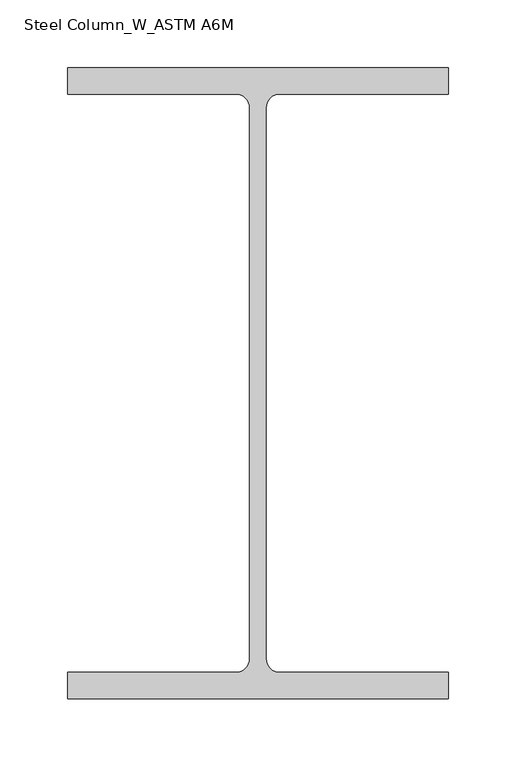
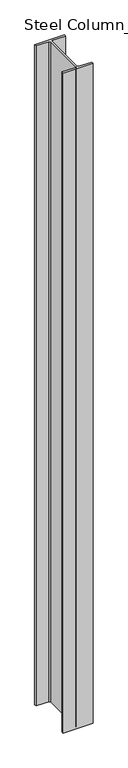
"""IFC4 building model written with IfcOpenShell, lengths in millimetres: column geometry, Steel Column_W_ASTM A6M : H_SC_AR_S01_W460x128_C1."""

from ifc_helpers import new_model, si_unit, point, frame, frame_2d, origin, place, context, project, spatial, polyline, circle_curve, trimmed, segment, composite_curve, outline, extrude, source, transform, mapped, element, save


def steel_column_w_astm_a6m_377c25c9(model_context):
    return source(origin(), model_context, "Body", "SweptSolid", [
        extrude(outline(composite_curve([segment(polyline([(141.0, 233.5), (141.0, 213.9), (16.2, 213.9)]), True, "CONTINUOUS"), segment(trimmed(circle_curve(frame_2d((16.2, 203.8)), 10.1), [point((16.2, 213.9))], [point((6.1, 203.8))], True, "CARTESIAN"), True, "CONTINUOUS"), segment(polyline([(6.1, 203.8), (6.1, -203.8)]), True, "CONTINUOUS"), segment(trimmed(circle_curve(frame_2d((16.2, -203.8)), 10.1), [point((6.1, -203.8))], [point((16.2, -213.9))], True, "CARTESIAN"), True, "CONTINUOUS"), segment(polyline([(16.2, -213.9), (141.0, -213.9), (141.0, -233.5), (-141.0, -233.5), (-141.0, -213.9), (-16.2, -213.9)]), True, "CONTINUOUS"), segment(trimmed(circle_curve(frame_2d((-16.2, -203.8)), 10.1), [point((-16.2, -213.9))], [point((-6.1, -203.8))], True, "CARTESIAN"), True, "CONTINUOUS"), segment(polyline([(-6.1, -203.8), (-6.1, 203.8)]), True, "CONTINUOUS"), segment(trimmed(circle_curve(frame_2d((-16.2, 203.8)), 10.1), [point((-6.1, 203.8))], [point((-16.2, 213.9))], True, "CARTESIAN"), True, "CONTINUOUS"), segment(polyline([(-16.2, 213.9), (-141.0, 213.9), (-141.0, 233.5), (141.0, 233.5)]), True, "CONTINUOUS")], self_intersect=False)), frame((0.0, 0.0, 3519.8243501), z_axis=(0.0, 0.0, 1.0), x_axis=(1.0, 0.0, 0.0)), (0.0, 0.0, 1.0), 6600.0),
    ])


if __name__ == "__main__":
    model = new_model("IFC4")
    model_context = context("Model", 3, world=origin())
    ifc_project = project(units=[si_unit("LENGTHUNIT", "METRE", prefix="MILLI")], contexts=[model_context])
    site = spatial("IfcSite", under=ifc_project)
    building = spatial("IfcBuilding", under=site)
    placement = place(None, origin())
    steel_column_w_astm_a6m_shape = steel_column_w_astm_a6m_377c25c9(model_context)
    element("IfcColumn", 1, ObjectType="Steel Column_W_ASTM A6M : H_SC_AR_S01_W460x128_C1", at=placement, inside=building, context=model_context, shape_type="MappedRepresentation", body=[
        mapped(steel_column_w_astm_a6m_shape, transform((0.0, 0.0, 0.0), x_axis=(1.0, 0.0, 0.0), y_axis=(0.0, 1.0, 0.0), z_axis=(0.0, 0.0, 1.0))),
    ])
    save(model, "model.ifc")

# Revit data of these elements
# Type "Steel Column_W_ASTM A6M : H_SC_AR_S01_W460x128_C1"
#   Section Name Key = "W18x86"
#   Width = 28.2 cm
#   Web Thickness = 1.22 cm
#   Web Fillet = 1.01 cm
#   Warping Constant = 3650000.0 cm⁶
#   Torsional Moment of Inertia = 171.00 cm⁴
#   Section Area = 163.0 cm²
#   Plastic Modulus weak axis = 793.0 cm³
#   Plastic Modulus strong axis = 3050.0 cm³
#   Perimeter = 2.02 m²/m
#   Nominal Weight = 128.00 kgf/m
#   Moment of Inertia weak axis = 7280.00 cm⁴
#   Moment of Inertia strong axis = 63700.00 cm⁴
#   Height = 46.7 cm
#   Flange Thickness = 1.96 cm
#   Elastic Modulus weak axis = 518.0 cm³
#   Elastic Modulus strong axis = 2720.0 cm³
#   Centroid Vertical = 23.35 cm
#   Centroid Horizontal = 14.1 cm
#   Structural Material [instance default] = Steel, 45-345
#   Bolt Spacing = 0
#   Assembly Code = ""
# Element 1 (IfcColumn, "Steel Column_W_ASTM A6M : H_SC_AR_S01_W460x128_C1")
#   Structural Material = Steel ASTM A992 GRADE 50
#   Materials on its faces: "Steel ASTM A992 GRADE 50"
# Materials
#   "Steel, 45-345": class "Metal", colour RGB 189 187 185, transparency 0, Description = "Steel 345 MPa", Cost = 0
#   "Steel ASTM A992 GRADE 50": class "Metal", colour RGB 120 120 120, transparency 0, Description = "Structural steel 50ksi", Cost = 0
